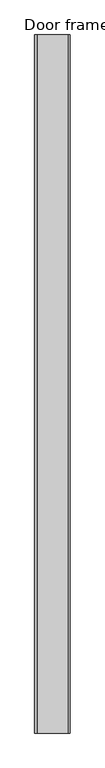
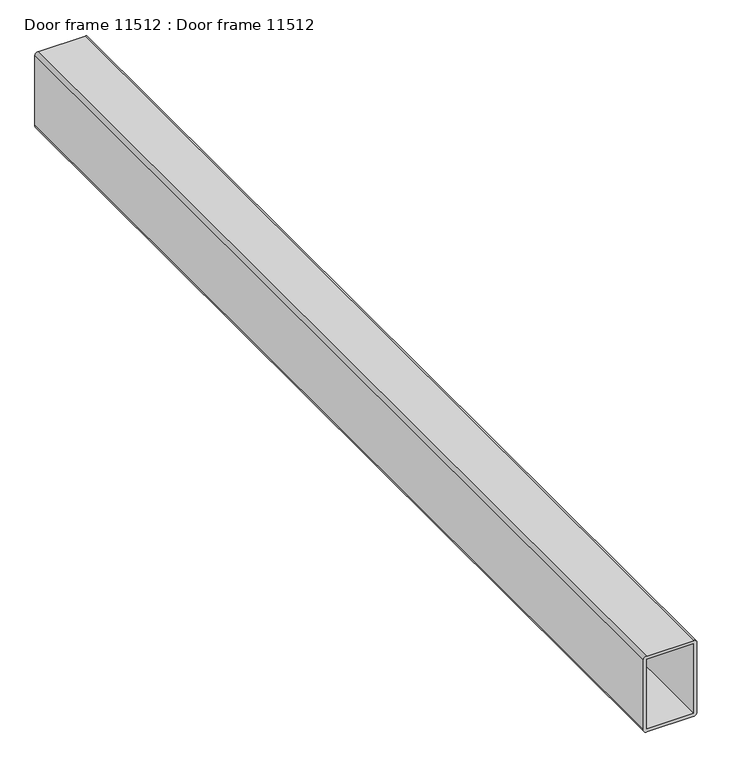
"""IFC4 building model written with IfcOpenShell, lengths in millimetres: proxy geometry, Door frame 11512 : Door frame 11512."""

from ifc_helpers import new_model, si_unit, point, frame, frame_2d, origin, place, context, project, spatial, polyline, circle_curve, trimmed, segment, composite_curve, outline, extrude, source, transform, mapped, element, save


def door_frame_11512_door_frame_11512_b90efb81(model_context):
    return source(origin(), model_context, "Body", "SweptSolid", [
        extrude(outline(composite_curve([segment(polyline([(34855.8775473, -8390.3106967), (34855.8775473, -8301.4106967)]), True, "CONTINUOUS"), segment(trimmed(circle_curve(frame_2d((34862.2275473, -8301.4106967)), 6.35), [point((34855.8775473, -8301.4106967))], [point((34862.2275473, -8295.0606967))], False, "CARTESIAN"), True, "CONTINUOUS"), segment(polyline([(34862.2275473, -8295.0606967), (35001.9275473, -8295.0606967)]), True, "CONTINUOUS"), segment(trimmed(circle_curve(frame_2d((35001.9275473, -8301.4106967)), 6.35), [point((35001.9275473, -8295.0606967))], [point((35008.2775473, -8301.4106967))], False, "CARTESIAN"), True, "CONTINUOUS"), segment(polyline([(35008.2775473, -8301.4106967), (35008.2775473, -8390.3106967)]), True, "CONTINUOUS"), segment(trimmed(circle_curve(frame_2d((35001.9275473, -8390.3106967)), 6.35), [point((35008.2775473, -8390.3106967))], [point((35001.9275473, -8396.6606967))], False, "CARTESIAN"), True, "CONTINUOUS"), segment(polyline([(35001.9275473, -8396.6606967), (34862.2275473, -8396.6606967)]), True, "CONTINUOUS"), segment(trimmed(circle_curve(frame_2d((34862.2275473, -8390.3106967)), 6.35), [point((34862.2275473, -8396.6606967))], [point((34855.8775473, -8390.3106967))], False, "CARTESIAN"), True, "CONTINUOUS")], self_intersect=False), holes=[polyline([(35001.7775473, -8301.5606967), (34862.3775473, -8301.5606967), (34862.3775473, -8390.1606967), (35001.7775473, -8390.1606967), (35001.7775473, -8301.5606967)])]), frame((0.0, 4540.4513244, 0.0), z_axis=(0.0, 1.0, 0.0), x_axis=(0.0, 0.0, 1.0)), (0.0, 0.0, 1.0), 2000.0),
    ])


if __name__ == "__main__":
    model = new_model("IFC4")
    model_context = context("Model", 3, world=origin())
    ifc_project = project(units=[si_unit("LENGTHUNIT", "METRE", prefix="MILLI")], contexts=[model_context])
    site = spatial("IfcSite", under=ifc_project)
    building = spatial("IfcBuilding", under=site)
    placement = place(None, origin())
    door_frame_11512_door_frame_11512_shape = door_frame_11512_door_frame_11512_b90efb81(model_context)
    element("IfcBuildingElementProxy", 1, Name="Door frame 11512 : Door frame 11512", ObjectType="Door frame 11512 : Door frame 11512", at=placement, inside=building, context=model_context, shape_type="MappedRepresentation", body=[
        mapped(door_frame_11512_door_frame_11512_shape, transform((0.0, 0.0, 0.0), x_axis=(1.0, 0.0, 0.0), y_axis=(0.0, 1.0, 0.0), z_axis=(0.0, 0.0, 1.0))),
    ])
    save(model, "model.ifc")

# Revit data of these elements
# Type "Door frame 11512 : Door frame 11512"
#   NameOverride = "Door frame"
# Element 1 (IfcBuildingElementProxy, "Door frame 11512 : Door frame 11512")
#   Materials on its faces: "DOOR FRAME: TUBE STEEL PROFILE - METALIZED, PRIMED & PAINTED (COLOR PER ARCHITECT)"
# Materials
#   "DOOR FRAME: TUBE STEEL PROFILE - METALIZED, PRIMED & PAINTED (COLOR PER ARCHITECT)": class "Unassigned", colour RGB 128 128 128, transparency 0, Cost = 0
